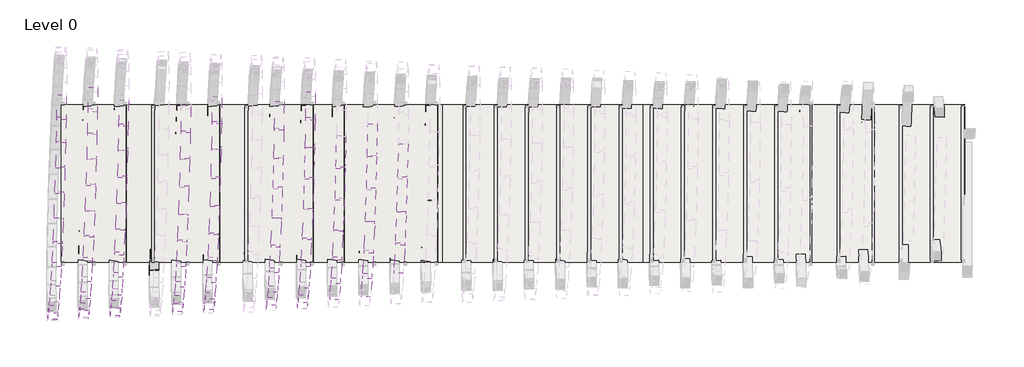
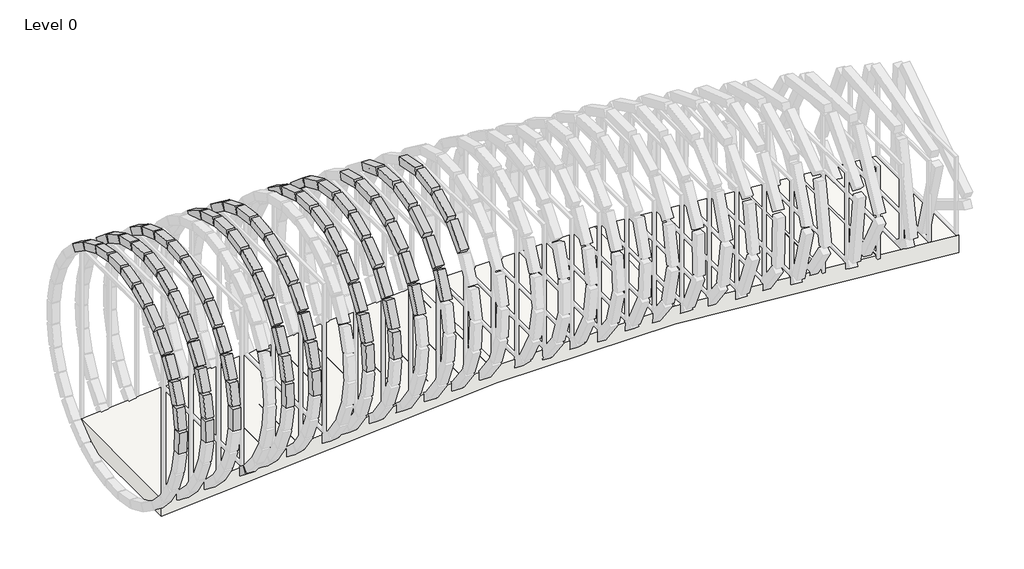
# One storey, part 1 of 6: 94 proxies, 1 slab.
# Revit data of these elements (continued)
# Project information
#   Project Issue Date = "Issue Date"
#   Project Status = "Project Status"
#   Client Name = "Owner"
#   Project Address = "Enter address here"
#   Project Name = "Project Name"
#   Project Number = "Project Number"
# Type "Family2 : Family2"
#   Default Elevation = 0
# Type "Floor-Grnd-Susp_65Scr-80Ins-100Blk-75PC"
#   Keynote = "E60/130"
#   Function = 0
#   Layers, outside or top first: 65 mm "Concrete, Sand/Cement Screed" (function 4); 0 mm "Vapor Retarder" (function 100); 80 mm "Rigid insulation" (function 3); 150 mm "Air" (function 3); 0 mm "Damp-proofing" (function 100); 100 mm "Concrete Masonry, Floor Block" (function 1); 75 mm "Concrete, Precast" (function 1)
# Elements 1, 2, 3, 4, 5, 6, 7, 8, 9, 10, 11, 12, 13, 14, 15, 16, 17, 18, 19, 20, 21, 22, 23, 24, 25, 26, 27, 28, 29, 30, 31, 32, 33, 34, 35, 36, 37, 38, 39, 40, 41, 42, 43, 44, 45, 46, 47, 48, 49, 50, 51, 52, 53, 54, 55, 56, 57, 58, 59, 60, 61, 62, 63, 64, 65, 66, 67, 68, 69, 70, 71, 72, 73, 74, 75, 76, 77, 78, 79, 80, 81, 82, 83, 84, 85, 86, 87, 88, 89, 90, 91, 92, 93, 94 (IfcBuildingElementProxy, "Family2 : Family2")
#   Phase Created = New Construction
# Element 95 (IfcSlab, "Floor-Grnd-Susp_65Scr-80Ins-100Blk-75PC")
#   Height Offset From Level = 0 mm
#   Phase Created = New Construction
#   Materials on its faces: "Concrete, Precast", "Concrete, Sand/Cement Screed"
# Materials
#   "Concrete, Sand/Cement Screed": class "Concrete", colour RGB 127 127 127, transparency 0, Description = "Concrete slab topping", Cost = 0
#   "Vapor Retarder": class "Generic", colour RGB 120 120 120, transparency 0, Description = "Polyethylene film membrane", Cost = 0
#   "Rigid insulation": class "Generic", colour RGB 127 127 127, transparency 0, Description = "Rigid foam insulation board", Cost = 0
#   "Air": class "Gas", colour RGB 255 255 255, transparency 0, Description = "Air", Cost = 0
#   "Damp-proofing": class "Generic", colour RGB 127 127 127, transparency 0, Description = "Damp-proofing", Cost = 0
#   "Concrete Masonry, Floor Block": class "Concrete", colour RGB 181 181 181, transparency 0, Description = "physical material", Cost = 0
#   "Concrete, Precast": class "Concrete", colour RGB 192 192 192, transparency 0, Description = "Precast concrete", Cost = 0
